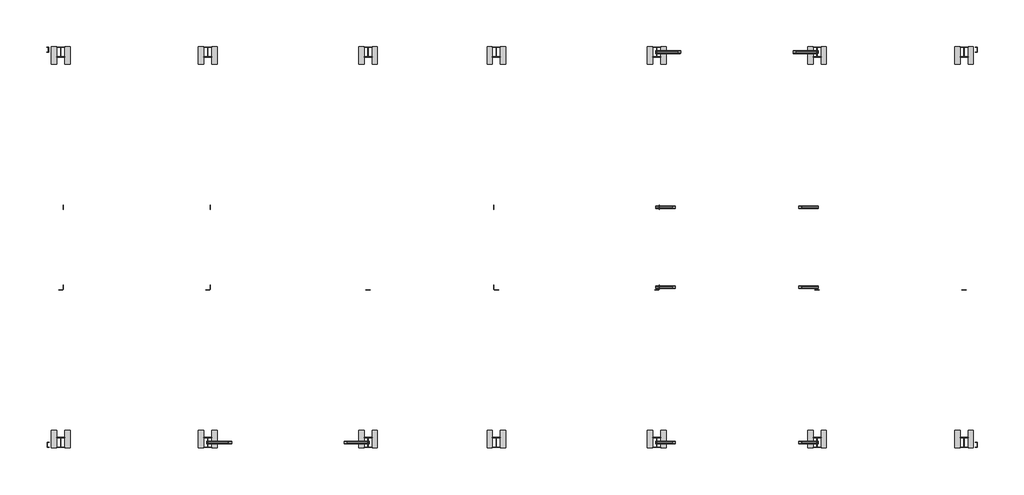
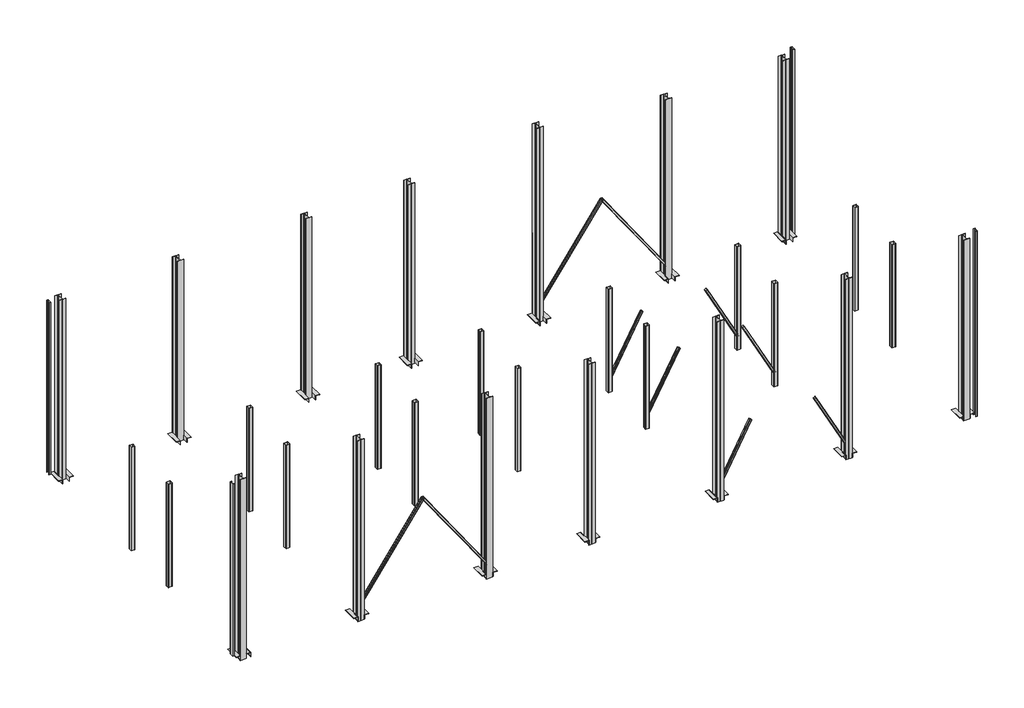
# One storey: 56 beams, 14 columns.
"""IFC4 building model written with IfcOpenShell, lengths in millimetres."""

import ifcopenshell
import ifcopenshell.guid

model = None  # the IFC model being written
_history = None  # IfcOwnerHistory: only IFC2X3 demands one
_inside = {}  # id of a spatial element -> (the spatial element, [elements in it])
_under = {}  # id of a project, library or spatial element -> (it, [spatial elements below it])
_declared = {}  # id of a project -> (the project, [libraries it declares])
_typed = {}  # id of a type object -> (the type object, [elements of that type])
_made_of = {}  # id of a material, layer set ... -> (it, [elements and type objects made of it])


def new_model(schema):
    """Start an empty IFC model of exactly this schema.

    Asked for "IFC4X3", IfcOpenShell would pick the latest addendum, in which some entities
    have other attributes; the version numbers below select the first issue.
    IFC2X3 requires an IfcOwnerHistory on every rooted entity: one is made here for all.
    """
    global model, _history
    if schema == "IFC4X3":
        model = ifcopenshell.file(schema_version=(4, 3, 0, 0))
    else:
        model = ifcopenshell.file(schema=schema)
    _inside.clear()
    _under.clear()
    _declared.clear()
    _typed.clear()
    _made_of.clear()
    _history = None
    if model.schema == "IFC2X3":
        org = make("IfcOrganization", Name="unknown")
        user = make(
            "IfcPersonAndOrganization",
            ThePerson=make("IfcPerson", FamilyName="unknown"),
            TheOrganization=org,
        )
        app = make(
            "IfcApplication",
            ApplicationDeveloper=org,
            Version="unknown",
            ApplicationFullName="unknown",
            ApplicationIdentifier="unknown",
        )
        _history = make(
            "IfcOwnerHistory",
            OwningUser=user,
            OwningApplication=app,
            ChangeAction="ADDED",
            CreationDate=0,
        )
    return model


def make(cls, **values):
    """One entity of the class cls with the attributes given. An attribute that is None is left unset."""
    return model.create_entity(
        cls, **{name: value for name, value in values.items() if value is not None}
    )


def rooted(cls, **values):
    """An entity with a GlobalId (a new one), such as an element, a storey or a relation."""
    return make(cls, GlobalId=ifcopenshell.guid.new(), OwnerHistory=_history, **values)


def si_unit(unit_type, name, prefix=None):
    """IfcSIUnit, for example si_unit("LENGTHUNIT", "METRE", prefix="MILLI")."""
    return make("IfcSIUnit", UnitType=unit_type, Prefix=prefix, Name=name)


def assignment(units):
    """IfcUnitAssignment: the units of a project."""
    return None if units is None else make("IfcUnitAssignment", Units=units)


def point(xyz):
    """IfcCartesianPoint."""
    return None if xyz is None else make("IfcCartesianPoint", Coordinates=xyz)


def direction(xyz):
    """IfcDirection."""
    return None if xyz is None else make("IfcDirection", DirectionRatios=xyz)


def frame(location, z_axis=None, x_axis=None):
    """IfcAxis2Placement3D, a coordinate frame: its origin and axes. An axis left out is left unset."""
    return make(
        "IfcAxis2Placement3D",
        Location=point(location),
        Axis=direction(z_axis),
        RefDirection=direction(x_axis),
    )


def frame_2d(location, x_axis=None):
    """IfcAxis2Placement2D, a coordinate frame in the plane: its origin and x axis."""
    return make(
        "IfcAxis2Placement2D", Location=point(location), RefDirection=direction(x_axis)
    )


def origin():
    """The frame at (0, 0, 0) with its axes left unset."""
    return frame((0.0, 0.0, 0.0))


def origin_with_axes():
    """The frame at (0, 0, 0) with the z axis (0, 0, 1) and the x axis (1, 0, 0) written out."""
    return frame((0.0, 0.0, 0.0), z_axis=(0.0, 0.0, 1.0), x_axis=(1.0, 0.0, 0.0))


def place(relative_to, where):
    """IfcLocalPlacement: puts the frame where relative to a parent placement (None: the world)."""
    return make(
        "IfcLocalPlacement", PlacementRelTo=relative_to, RelativePlacement=where
    )


def context(
    kind, dimensions, precision=None, world=None, true_north=None, identifier=None
):
    """IfcGeometricRepresentationContext, for example the 3D "Model" context."""
    return make(
        "IfcGeometricRepresentationContext",
        ContextIdentifier=identifier,
        ContextType=kind,
        CoordinateSpaceDimension=dimensions,
        Precision=precision,
        WorldCoordinateSystem=world,
        TrueNorth=true_north,
    )


def project(units=None, contexts=None):
    """IfcProject with its units and contexts."""
    return rooted(
        "IfcProject",
        Name="project",
        RepresentationContexts=contexts,
        UnitsInContext=assignment(units),
    )


def spatial(cls, under=None, at=None, **own):
    """A site, building, storey or space (cls), placed at a placement, below another one or the project."""
    s = rooted(cls, ObjectPlacement=at, **own)
    if under is not None:
        _under.setdefault(under.id(), (under, []))[1].append(s)
    return s


def polyline(points):
    """IfcPolyline through the points."""
    return make("IfcPolyline", Points=[point(p) for p in points])


def circle_curve(where, radius):
    """IfcCircle in the frame where."""
    return make("IfcCircle", Position=where, Radius=radius)


def trimmed(basis, trim1, trim2, sense, master):
    """IfcTrimmedCurve: the piece of a basis curve between two trims."""
    return make(
        "IfcTrimmedCurve",
        BasisCurve=basis,
        Trim1=trim1,
        Trim2=trim2,
        SenseAgreement=sense,
        MasterRepresentation=master,
    )


def segment(curve, same_sense, transition):
    """IfcCompositeCurveSegment."""
    return make(
        "IfcCompositeCurveSegment",
        Transition=transition,
        SameSense=same_sense,
        ParentCurve=curve,
    )


def composite_curve(segments, self_intersect=None):
    """IfcCompositeCurve: segments joined end to end."""
    return make("IfcCompositeCurve", Segments=segments, SelfIntersect=self_intersect)


def outline(outer, holes=None, kind="AREA"):
    """IfcArbitraryClosedProfileDef: a profile drawn as a closed curve; with holes, ...WithVoids."""
    if holes is None:
        return make("IfcArbitraryClosedProfileDef", ProfileType=kind, OuterCurve=outer)
    return make(
        "IfcArbitraryProfileDefWithVoids",
        ProfileType=kind,
        OuterCurve=outer,
        InnerCurves=holes,
    )


def extrude(swept, where, along, depth):
    """IfcExtrudedAreaSolid: the profile swept, set in the frame where, extruded along a direction by depth."""
    return make(
        "IfcExtrudedAreaSolid",
        SweptArea=swept,
        Position=where,
        ExtrudedDirection=direction(along),
        Depth=depth,
    )


def shape(context_of_items, identifier, shape_type, items):
    """IfcShapeRepresentation: the items that make up one representation, for example the "Body"."""
    return make(
        "IfcShapeRepresentation",
        ContextOfItems=context_of_items,
        RepresentationIdentifier=identifier,
        RepresentationType=shape_type,
        Items=items,
    )


def source(mapping_origin, context_of_items, identifier, shape_type, items):
    """IfcRepresentationMap: a shape defined once, which mapped items show again and again."""
    return make(
        "IfcRepresentationMap",
        MappingOrigin=mapping_origin,
        MappedRepresentation=shape(context_of_items, identifier, shape_type, items),
    )


def transform(
    local_origin,
    x_axis=None,
    y_axis=None,
    z_axis=None,
    scale=None,
    scale2=None,
    scale3=None,
    uniform=True,
):
    """IfcCartesianTransformationOperator3D, or its non-uniform kind. x_axis, y_axis, z_axis: its Axis1, 2, 3."""
    if uniform:
        return make(
            "IfcCartesianTransformationOperator3D",
            Axis1=direction(x_axis),
            Axis2=direction(y_axis),
            LocalOrigin=point(local_origin),
            Scale=scale,
            Axis3=direction(z_axis),
        )
    return make(
        "IfcCartesianTransformationOperator3DnonUniform",
        Axis1=direction(x_axis),
        Axis2=direction(y_axis),
        LocalOrigin=point(local_origin),
        Scale=scale,
        Axis3=direction(z_axis),
        Scale2=scale2,
        Scale3=scale3,
    )


def mapped(mapping_source, mapping_target):
    """IfcMappedItem: shows the shape of a source again, moved by a transform."""
    return make(
        "IfcMappedItem", MappingSource=mapping_source, MappingTarget=mapping_target
    )


def made_of(thing, what):
    """Note that an element or type object is made of a material, layer set ...; save() writes the relation."""
    if what is not None:
        _made_of.setdefault(what.id(), (what, []))[1].append(thing)
    return thing


def element(
    cls,
    number,
    at=None,
    inside=None,
    cuts=None,
    type_object=None,
    material=None,
    context=None,
    identifier="Body",
    shape_type=None,
    held_by="IfcProductDefinitionShape",
    body=None,
    shapes=None,
    **own,
):
    """One element of the class cls, such as IfcWall. Its Tag is "e" and its number.

    at: its placement. inside: the storey or other place that contains it. cuts: it is an
    opening in that element (IfcRelVoidsElement). A single representation is given by context,
    identifier, shape_type and body (its items); several are given by shapes. held_by: the class
    of the entity that holds the representations. save() writes the other relations.
    """
    e = rooted(cls, Tag="e%d" % number, ObjectPlacement=at, **own)
    if body is not None:
        shapes = [shape(context, identifier, shape_type, body)]
    if shapes is not None:
        e.Representation = make(held_by, Representations=shapes)
    if inside is not None:
        _inside.setdefault(inside.id(), (inside, []))[1].append(e)
    if cuts is not None:
        rooted(
            "IfcRelVoidsElement", RelatingBuildingElement=cuts, RelatedOpeningElement=e
        )
    if type_object is not None:
        _typed.setdefault(type_object.id(), (type_object, []))[1].append(e)
    return made_of(e, material)


def aggregate(whole, parts):
    """IfcRelAggregates: a whole, such as a stair, and the parts it consists of."""
    return rooted("IfcRelAggregates", RelatingObject=whole, RelatedObjects=parts)


def save(model, path):
    """Write the relations noted so far, then the file.

    IfcRelAggregates (storeys below a building ...), IfcRelContainedInSpatialStructure (elements
    in a storey), IfcRelDefinesByType, IfcRelAssociatesMaterial and IfcRelDeclares: one each for
    every whole, place, type object, material and project.
    """
    for whole, parts in _under.values():
        aggregate(whole, parts)
    for where, things in _inside.values():
        rooted(
            "IfcRelContainedInSpatialStructure",
            RelatedElements=things,
            RelatingStructure=where,
        )
    for kind, things in _typed.values():
        rooted("IfcRelDefinesByType", RelatedObjects=things, RelatingType=kind)
    for what, things in _made_of.values():
        rooted("IfcRelAssociatesMaterial", RelatedObjects=things, RelatingMaterial=what)
    for by, libraries in _declared.values():
        rooted("IfcRelDeclares", RelatingContext=by, RelatedDefinitions=libraries)
    model.write(path)


def beam_75da4e79(model_context):
    return source(origin(), model_context, "Body", "SweptSolid", [
        extrude(outline(composite_curve([segment(polyline([(-78.0, 90.0), (78.0, 90.0)]), True, "CONTINUOUS"), segment(trimmed(circle_curve(frame_2d((78.0, 78.0)), 12.0), [point((78.0, 90.0))], [point((90.0, 78.0))], False, "CARTESIAN"), True, "CONTINUOUS"), segment(polyline([(90.0, 78.0), (90.0, -78.0)]), True, "CONTINUOUS"), segment(trimmed(circle_curve(frame_2d((78.0, -78.0)), 12.0), [point((90.0, -78.0))], [point((78.0, -90.0))], False, "CARTESIAN"), True, "CONTINUOUS"), segment(polyline([(78.0, -90.0), (-78.0, -90.0)]), True, "CONTINUOUS"), segment(trimmed(circle_curve(frame_2d((-78.0, -78.0)), 12.0), [point((-78.0, -90.0))], [point((-90.0, -78.0))], False, "CARTESIAN"), True, "CONTINUOUS"), segment(polyline([(-90.0, -78.0), (-90.0, 78.0)]), True, "CONTINUOUS"), segment(trimmed(circle_curve(frame_2d((-78.0, 78.0)), 12.0), [point((-90.0, 78.0))], [point((-78.0, 90.0))], False, "CARTESIAN"), True, "CONTINUOUS")], self_intersect=False), holes=[composite_curve([segment(trimmed(circle_curve(frame_2d((-78.0, 78.0)), 6.0), [point((-78.0, 84.0))], [point((-84.0, 78.0))], True, "CARTESIAN"), True, "CONTINUOUS"), segment(polyline([(-84.0, 78.0), (-84.0, -78.0)]), True, "CONTINUOUS"), segment(trimmed(circle_curve(frame_2d((-78.0, -78.0)), 6.0), [point((-84.0, -78.0))], [point((-78.0, -84.0))], True, "CARTESIAN"), True, "CONTINUOUS"), segment(polyline([(-78.0, -84.0), (78.0, -84.0)]), True, "CONTINUOUS"), segment(trimmed(circle_curve(frame_2d((78.0, -78.0)), 6.0), [point((78.0, -84.0))], [point((84.0, -78.0))], True, "CARTESIAN"), True, "CONTINUOUS"), segment(polyline([(84.0, -78.0), (84.0, 78.0)]), True, "CONTINUOUS"), segment(trimmed(circle_curve(frame_2d((78.0, 78.0)), 6.0), [point((84.0, 78.0))], [point((78.0, 84.0))], True, "CARTESIAN"), True, "CONTINUOUS"), segment(polyline([(78.0, 84.0), (-78.0, 84.0)]), True, "CONTINUOUS")], self_intersect=False)]), frame((-2550.0, 0.0, 0.0), z_axis=(1.0, 0.0, 0.0), x_axis=(0.0, 1.0, 0.0)), (0.0, 0.0, 1.0), 5100.0),
    ])


def beam_97961db2(model_context):
    return source(origin(), model_context, "Body", "SweptSolid", [
        extrude(outline(composite_curve([segment(polyline([(23.0, 100.0), (23.0, -100.0), (-53.0, -100.0), (-53.0, -91.0), (8.3, -91.0)]), True, "CONTINUOUS"), segment(trimmed(circle_curve(frame_2d((8.3, -81.5)), 9.5), [point((8.3, -91.0))], [point((17.8, -81.5))], True, "CARTESIAN"), True, "CONTINUOUS"), segment(polyline([(17.8, -81.5), (17.8, 81.5)]), True, "CONTINUOUS"), segment(trimmed(circle_curve(frame_2d((8.3, 81.5)), 9.5), [point((17.8, 81.5))], [point((8.3, 91.0))], True, "CARTESIAN"), True, "CONTINUOUS"), segment(polyline([(8.3, 91.0), (-53.0, 91.0), (-53.0, 100.0), (23.0, 100.0)]), True, "CONTINUOUS")], self_intersect=False)), frame((-4250.0, 0.0, 0.0), z_axis=(1.0, 0.0, 0.0), x_axis=(0.0, 1.0, 0.0)), (0.0, 0.0, 1.0), 8500.0),
    ])


def beam_6aa5ee4f(model_context):
    return source(origin(), model_context, "Body", "SweptSolid", [
        extrude(outline(composite_curve([segment(polyline([(-38.0, 50.0), (38.0, 50.0)]), True, "CONTINUOUS"), segment(trimmed(circle_curve(frame_2d((38.0, 38.0)), 12.0), [point((38.0, 50.0))], [point((50.0, 38.0))], False, "CARTESIAN"), True, "CONTINUOUS"), segment(polyline([(50.0, 38.0), (50.0, -38.0)]), True, "CONTINUOUS"), segment(trimmed(circle_curve(frame_2d((38.0, -38.0)), 12.0), [point((50.0, -38.0))], [point((38.0, -50.0))], False, "CARTESIAN"), True, "CONTINUOUS"), segment(polyline([(38.0, -50.0), (-38.0, -50.0)]), True, "CONTINUOUS"), segment(trimmed(circle_curve(frame_2d((-38.0, -38.0)), 12.0), [point((-38.0, -50.0))], [point((-50.0, -38.0))], False, "CARTESIAN"), True, "CONTINUOUS"), segment(polyline([(-50.0, -38.0), (-50.0, 38.0)]), True, "CONTINUOUS"), segment(trimmed(circle_curve(frame_2d((-38.0, 38.0)), 12.0), [point((-50.0, 38.0))], [point((-38.0, 50.0))], False, "CARTESIAN"), True, "CONTINUOUS")], self_intersect=False), holes=[composite_curve([segment(trimmed(circle_curve(frame_2d((-38.0, 38.0)), 6.0), [point((-38.0, 44.0))], [point((-44.0, 38.0))], True, "CARTESIAN"), True, "CONTINUOUS"), segment(polyline([(-44.0, 38.0), (-44.0, -38.0)]), True, "CONTINUOUS"), segment(trimmed(circle_curve(frame_2d((-38.0, -38.0)), 6.0), [point((-44.0, -38.0))], [point((-38.0, -44.0))], True, "CARTESIAN"), True, "CONTINUOUS"), segment(polyline([(-38.0, -44.0), (38.0, -44.0)]), True, "CONTINUOUS"), segment(trimmed(circle_curve(frame_2d((38.0, -38.0)), 6.0), [point((38.0, -44.0))], [point((44.0, -38.0))], True, "CARTESIAN"), True, "CONTINUOUS"), segment(polyline([(44.0, -38.0), (44.0, 38.0)]), True, "CONTINUOUS"), segment(trimmed(circle_curve(frame_2d((38.0, 38.0)), 6.0), [point((44.0, 38.0))], [point((38.0, 44.0))], True, "CARTESIAN"), True, "CONTINUOUS"), segment(polyline([(38.0, 44.0), (-38.0, 44.0)]), True, "CONTINUOUS")], self_intersect=False)]), frame((-2618.5, 0.0, 0.0), z_axis=(1.0, 0.0, 0.0), x_axis=(0.0, 1.0, 0.0)), (0.0, 0.0, 1.0), 5237.0),
    ])


def beam_810e5c83(model_context):
    return source(origin(), model_context, "Body", "SweptSolid", [
        extrude(outline(composite_curve([segment(polyline([(-38.0, 50.0), (38.0, 50.0)]), True, "CONTINUOUS"), segment(trimmed(circle_curve(frame_2d((38.0, 38.0)), 12.0), [point((38.0, 50.0))], [point((50.0, 38.0))], False, "CARTESIAN"), True, "CONTINUOUS"), segment(polyline([(50.0, 38.0), (50.0, -38.0)]), True, "CONTINUOUS"), segment(trimmed(circle_curve(frame_2d((38.0, -38.0)), 12.0), [point((50.0, -38.0))], [point((38.0, -50.0))], False, "CARTESIAN"), True, "CONTINUOUS"), segment(polyline([(38.0, -50.0), (-38.0, -50.0)]), True, "CONTINUOUS"), segment(trimmed(circle_curve(frame_2d((-38.0, -38.0)), 12.0), [point((-38.0, -50.0))], [point((-50.0, -38.0))], False, "CARTESIAN"), True, "CONTINUOUS"), segment(polyline([(-50.0, -38.0), (-50.0, 38.0)]), True, "CONTINUOUS"), segment(trimmed(circle_curve(frame_2d((-38.0, 38.0)), 12.0), [point((-50.0, 38.0))], [point((-38.0, 50.0))], False, "CARTESIAN"), True, "CONTINUOUS")], self_intersect=False), holes=[composite_curve([segment(trimmed(circle_curve(frame_2d((-38.0, 38.0)), 6.0), [point((-38.0, 44.0))], [point((-44.0, 38.0))], True, "CARTESIAN"), True, "CONTINUOUS"), segment(polyline([(-44.0, 38.0), (-44.0, -38.0)]), True, "CONTINUOUS"), segment(trimmed(circle_curve(frame_2d((-38.0, -38.0)), 6.0), [point((-44.0, -38.0))], [point((-38.0, -44.0))], True, "CARTESIAN"), True, "CONTINUOUS"), segment(polyline([(-38.0, -44.0), (38.0, -44.0)]), True, "CONTINUOUS"), segment(trimmed(circle_curve(frame_2d((38.0, -38.0)), 6.0), [point((38.0, -44.0))], [point((44.0, -38.0))], True, "CARTESIAN"), True, "CONTINUOUS"), segment(polyline([(44.0, -38.0), (44.0, 38.0)]), True, "CONTINUOUS"), segment(trimmed(circle_curve(frame_2d((38.0, 38.0)), 6.0), [point((44.0, 38.0))], [point((38.0, 44.0))], True, "CARTESIAN"), True, "CONTINUOUS"), segment(polyline([(38.0, 44.0), (-38.0, 44.0)]), True, "CONTINUOUS")], self_intersect=False)]), frame((-1601.0, 0.0, 0.0), z_axis=(1.0, 0.0, 0.0), x_axis=(0.0, 1.0, 0.0)), (0.0, 0.0, 1.0), 3202.0),
    ])


def beam_48740a10(model_context):
    return source(origin(), model_context, "Body", "SweptSolid", [
        extrude(outline(composite_curve([segment(polyline([(-23.0, 100.0), (53.0, 100.0), (53.0, 91.0), (-8.3, 91.0)]), True, "CONTINUOUS"), segment(trimmed(circle_curve(frame_2d((-8.3, 81.5)), 9.5), [point((-8.3, 91.0))], [point((-17.8, 81.5))], True, "CARTESIAN"), True, "CONTINUOUS"), segment(polyline([(-17.8, 81.5), (-17.8, -81.5)]), True, "CONTINUOUS"), segment(trimmed(circle_curve(frame_2d((-8.3, -81.5)), 9.5), [point((-17.8, -81.5))], [point((-8.3, -91.0))], True, "CARTESIAN"), True, "CONTINUOUS"), segment(polyline([(-8.3, -91.0), (53.0, -91.0), (53.0, -100.0), (-23.0, -100.0), (-23.0, 100.0)]), True, "CONTINUOUS")], self_intersect=False)), frame((-4585.0, 0.0, 0.0), z_axis=(1.0, 0.0, 0.0), x_axis=(0.0, 1.0, 0.0)), (0.0, 0.0, 1.0), 9170.0),
    ])


def beam_e8fb0e59(model_context):
    return source(origin(), model_context, "Body", "SweptSolid", [
        extrude(outline(composite_curve([segment(polyline([(23.0, 100.0), (23.0, -100.0), (-53.0, -100.0), (-53.0, -91.0), (8.3, -91.0)]), True, "CONTINUOUS"), segment(trimmed(circle_curve(frame_2d((8.3, -81.5)), 9.5), [point((8.3, -91.0))], [point((17.8, -81.5))], True, "CARTESIAN"), True, "CONTINUOUS"), segment(polyline([(17.8, -81.5), (17.8, 81.5)]), True, "CONTINUOUS"), segment(trimmed(circle_curve(frame_2d((8.3, 81.5)), 9.5), [point((17.8, 81.5))], [point((8.3, 91.0))], True, "CARTESIAN"), True, "CONTINUOUS"), segment(polyline([(8.3, 91.0), (-53.0, 91.0), (-53.0, 100.0), (23.0, 100.0)]), True, "CONTINUOUS")], self_intersect=False)), frame((-4585.0, 0.0, 0.0), z_axis=(1.0, 0.0, 0.0), x_axis=(0.0, 1.0, 0.0)), (0.0, 0.0, 1.0), 9170.0),
    ])


def l_200x14_1023fe27(model_context):
    return source(origin(), model_context, "Body", "SweptSolid", [
        extrude(outline(composite_curve([segment(polyline([(54.6, -54.6), (-145.4, -54.6), (-145.4, -46.6)]), True, "CONTINUOUS"), segment(trimmed(circle_curve(frame_2d((-139.4, -46.6)), 6.0), [point((-145.4, -46.6))], [point((-139.4, -40.6))], False, "CARTESIAN"), True, "CONTINUOUS"), segment(polyline([(-139.4, -40.6), (22.6, -40.6)]), True, "CONTINUOUS"), segment(trimmed(circle_curve(frame_2d((22.6, -22.6)), 18.0), [point((22.6, -40.6))], [point((40.6, -22.6))], True, "CARTESIAN"), True, "CONTINUOUS"), segment(polyline([(40.6, -22.6), (40.6, 139.4)]), True, "CONTINUOUS"), segment(trimmed(circle_curve(frame_2d((46.6, 139.4)), 6.0), [point((40.6, 139.4))], [point((46.6, 145.4))], False, "CARTESIAN"), True, "CONTINUOUS"), segment(polyline([(46.6, 145.4), (54.6, 145.4), (54.6, -54.6)]), True, "CONTINUOUS")], self_intersect=False)), frame((-335.0, 0.0, 0.0), z_axis=(1.0, 0.0, 0.0), x_axis=(0.0, 1.0, 0.0)), (0.0, 0.0, 1.0), 670.0),
    ])


def l_200x14_4beb5e8d(model_context):
    return source(origin(), model_context, "Body", "SweptSolid", [
        extrude(outline(composite_curve([segment(polyline([(-54.6, -54.6), (-54.6, 145.4), (-46.6, 145.4)]), True, "CONTINUOUS"), segment(trimmed(circle_curve(frame_2d((-46.6, 139.4)), 6.0), [point((-46.6, 145.4))], [point((-40.6, 139.4))], False, "CARTESIAN"), True, "CONTINUOUS"), segment(polyline([(-40.6, 139.4), (-40.6, -22.6)]), True, "CONTINUOUS"), segment(trimmed(circle_curve(frame_2d((-22.6, -22.6)), 18.0), [point((-40.6, -22.6))], [point((-22.6, -40.6))], True, "CARTESIAN"), True, "CONTINUOUS"), segment(polyline([(-22.6, -40.6), (139.4, -40.6)]), True, "CONTINUOUS"), segment(trimmed(circle_curve(frame_2d((139.4, -46.6)), 6.0), [point((139.4, -40.6))], [point((145.4, -46.6))], False, "CARTESIAN"), True, "CONTINUOUS"), segment(polyline([(145.4, -46.6), (145.4, -54.6), (-54.6, -54.6)]), True, "CONTINUOUS")], self_intersect=False)), frame((-335.0, 0.0, 0.0), z_axis=(1.0, 0.0, 0.0), x_axis=(0.0, 1.0, 0.0)), (0.0, 0.0, 1.0), 670.0),
    ])


def i_40h1_838be756(model_context):
    return source(origin(), model_context, "Body", "SweptSolid", [
        extrude(outline(composite_curve([segment(polyline([(-149.5, -178.5), (-26.75, -178.5)]), True, "CONTINUOUS"), segment(trimmed(circle_curve(frame_2d((-26.75, -156.5)), 22.0), [point((-26.75, -178.5))], [point((-4.75, -156.5))], True, "CARTESIAN"), True, "CONTINUOUS"), segment(polyline([(-4.75, -156.5), (-4.75, 157.5)]), True, "CONTINUOUS"), segment(trimmed(circle_curve(frame_2d((-26.75, 157.5)), 22.0), [point((-4.75, 157.5))], [point((-26.75, 179.5))], True, "CARTESIAN"), True, "CONTINUOUS"), segment(polyline([(-26.75, 179.5), (-149.5, 179.5), (-149.5, 192.0), (149.5, 192.0), (149.5, 179.5), (26.75, 179.5)]), True, "CONTINUOUS"), segment(trimmed(circle_curve(frame_2d((26.75, 157.5)), 22.0), [point((26.75, 179.5))], [point((4.75, 157.5))], True, "CARTESIAN"), True, "CONTINUOUS"), segment(polyline([(4.75, 157.5), (4.75, -156.5)]), True, "CONTINUOUS"), segment(trimmed(circle_curve(frame_2d((26.75, -156.5)), 22.0), [point((4.75, -156.5))], [point((26.75, -178.5))], True, "CARTESIAN"), True, "CONTINUOUS"), segment(polyline([(26.75, -178.5), (149.5, -178.5), (149.5, -191.0), (-149.5, -191.0), (-149.5, -178.5)]), True, "CONTINUOUS")], self_intersect=False)), origin_with_axes(), (0.0, 0.0, 1.0), 9604.6332616),
    ])


def i_40h1_0f399548(model_context):
    return source(origin(), model_context, "Body", "SweptSolid", [
        extrude(outline(composite_curve([segment(polyline([(-149.5, 178.5), (-149.5, 191.0), (149.5, 191.0), (149.5, 178.5), (26.75, 178.5)]), True, "CONTINUOUS"), segment(trimmed(circle_curve(frame_2d((26.75, 156.5)), 22.0), [point((26.75, 178.5))], [point((4.75, 156.5))], True, "CARTESIAN"), True, "CONTINUOUS"), segment(polyline([(4.75, 156.5), (4.75, -157.5)]), True, "CONTINUOUS"), segment(trimmed(circle_curve(frame_2d((26.75, -157.5)), 22.0), [point((4.75, -157.5))], [point((26.75, -179.5))], True, "CARTESIAN"), True, "CONTINUOUS"), segment(polyline([(26.75, -179.5), (149.5, -179.5), (149.5, -192.0), (-149.5, -192.0), (-149.5, -179.5), (-26.75, -179.5)]), True, "CONTINUOUS"), segment(trimmed(circle_curve(frame_2d((-26.75, -157.5)), 22.0), [point((-26.75, -179.5))], [point((-4.75, -157.5))], True, "CARTESIAN"), True, "CONTINUOUS"), segment(polyline([(-4.75, -157.5), (-4.75, 156.5)]), True, "CONTINUOUS"), segment(trimmed(circle_curve(frame_2d((-26.75, 156.5)), 22.0), [point((-4.75, 156.5))], [point((-26.75, 178.5))], True, "CARTESIAN"), True, "CONTINUOUS"), segment(polyline([(-26.75, 178.5), (-149.5, 178.5)]), True, "CONTINUOUS")], self_intersect=False)), origin_with_axes(), (0.0, 0.0, 1.0), 8923.3858447),
    ])


def i_40h1_edde52e3(model_context):
    return source(origin(), model_context, "Body", "SweptSolid", [
        extrude(outline(composite_curve([segment(polyline([(-149.5, -178.5), (-26.75, -178.5)]), True, "CONTINUOUS"), segment(trimmed(circle_curve(frame_2d((-26.75, -156.5)), 22.0), [point((-26.75, -178.5))], [point((-4.75, -156.5))], True, "CARTESIAN"), True, "CONTINUOUS"), segment(polyline([(-4.75, -156.5), (-4.75, 157.5)]), True, "CONTINUOUS"), segment(trimmed(circle_curve(frame_2d((-26.75, 157.5)), 22.0), [point((-4.75, 157.5))], [point((-26.75, 179.5))], True, "CARTESIAN"), True, "CONTINUOUS"), segment(polyline([(-26.75, 179.5), (-149.5, 179.5), (-149.5, 192.0), (149.5, 192.0), (149.5, 179.5), (26.75, 179.5)]), True, "CONTINUOUS"), segment(trimmed(circle_curve(frame_2d((26.75, 157.5)), 22.0), [point((26.75, 179.5))], [point((4.75, 157.5))], True, "CARTESIAN"), True, "CONTINUOUS"), segment(polyline([(4.75, 157.5), (4.75, -156.5)]), True, "CONTINUOUS"), segment(trimmed(circle_curve(frame_2d((26.75, -156.5)), 22.0), [point((4.75, -156.5))], [point((26.75, -178.5))], True, "CARTESIAN"), True, "CONTINUOUS"), segment(polyline([(26.75, -178.5), (149.5, -178.5), (149.5, -191.0), (-149.5, -191.0), (-149.5, -178.5)]), True, "CONTINUOUS")], self_intersect=False)), origin_with_axes(), (0.0, 0.0, 1.0), 8923.3858447),
    ])


model = new_model("IFC4")

# Units and contexts
model_context = context("Model", 3, world=origin())
ifc_project = project(units=[si_unit("LENGTHUNIT", "METRE", prefix="MILLI")], contexts=[model_context])

# Site, building, storey
site = spatial("IfcSite", under=ifc_project)
building = spatial("IfcBuilding", under=site)
storey = spatial("IfcBuildingStorey", under=building, Name="Этаж 01", Elevation=0.0)

# Beams
placement = place(None, origin())
beam_shape = beam_75da4e79(model_context)
element("IfcBeam", 1, ObjectType="Гнутый прямоугольный профиль (Трубы 30245-94) Балки : гнутый прямоуг. проф. 180x6", at=placement, inside=storey, context=model_context, shape_type="MappedRepresentation", body=[
    mapped(beam_shape, transform((6000.0, 9000.0, 1950.0), x_axis=(0.0, 0.0, 1.0), y_axis=(0.0, -1.0, 0.0), z_axis=(1.0, 0.0, 0.0))),
])
element("IfcBeam", 2, ObjectType="Гнутый прямоугольный профиль (Трубы 30245-94) Балки : гнутый прямоуг. проф. 180x6", at=placement, inside=storey, context=model_context, shape_type="MappedRepresentation", body=[
    mapped(beam_shape, transform((6000.0, 6000.0, 1950.0), x_axis=(0.0, 0.0, 1.0), y_axis=(0.0, -1.0, 0.0), z_axis=(1.0, 0.0, 0.0))),
])
element("IfcBeam", 3, ObjectType="Гнутый прямоугольный профиль (Трубы 30245-94) Балки : гнутый прямоуг. проф. 180x6", at=placement, inside=storey, context=model_context, shape_type="MappedRepresentation", body=[
    mapped(beam_shape, transform((12000.0, 9000.0, 1950.0), x_axis=(0.0, 0.0, 1.0), y_axis=(0.0, -1.0, 0.0), z_axis=(1.0, 0.0, 0.0))),
])
element("IfcBeam", 4, ObjectType="Гнутый прямоугольный профиль (Трубы 30245-94) Балки : гнутый прямоуг. проф. 180x6", at=placement, inside=storey, context=model_context, shape_type="MappedRepresentation", body=[
    mapped(beam_shape, transform((12000.0, 6000.0, 1950.0), x_axis=(0.0, 0.0, 1.0), y_axis=(0.0, -1.0, 0.0), z_axis=(1.0, 0.0, 0.0))),
])
element("IfcBeam", 5, ObjectType="Гнутый прямоугольный профиль (Трубы 30245-94) Балки : гнутый прямоуг. проф. 180x6", at=placement, inside=storey, context=model_context, shape_type="MappedRepresentation", body=[
    mapped(beam_shape, transform((16800.0, 9000.0, 1950.0), x_axis=(0.0, 0.0, 1.0), y_axis=(0.0, -1.0, 0.0), z_axis=(1.0, 0.0, 0.0))),
])
element("IfcBeam", 6, ObjectType="Гнутый прямоугольный профиль (Трубы 30245-94) Балки : гнутый прямоуг. проф. 180x6", at=placement, inside=storey, context=model_context, shape_type="MappedRepresentation", body=[
    mapped(beam_shape, transform((16800.0, 6000.0, 1950.0), x_axis=(0.0, 0.0, 1.0), y_axis=(0.0, -1.0, 0.0), z_axis=(1.0, 0.0, 0.0))),
])
element("IfcBeam", 7, ObjectType="Гнутый прямоугольный профиль (Трубы 30245-94) Балки : гнутый прямоуг. проф. 180x6", at=placement, inside=storey, context=model_context, shape_type="MappedRepresentation", body=[
    mapped(beam_shape, transform((22800.0, 9000.0, 1950.0), x_axis=(0.0, 0.0, 1.0), y_axis=(0.0, -1.0, 0.0), z_axis=(1.0, 0.0, 0.0))),
])
element("IfcBeam", 8, ObjectType="Гнутый прямоугольный профиль (Трубы 30245-94) Балки : гнутый прямоуг. проф. 180x6", at=placement, inside=storey, context=model_context, shape_type="MappedRepresentation", body=[
    mapped(beam_shape, transform((22800.0, 6000.0, 1950.0), x_axis=(0.0, 0.0, 1.0), y_axis=(0.0, -1.0, 0.0), z_axis=(1.0, 0.0, 0.0))),
])
element("IfcBeam", 9, ObjectType="Гнутый прямоугольный профиль (Трубы 30245-94) Балки : гнутый прямоуг. проф. 180x6", at=placement, inside=storey, context=model_context, shape_type="MappedRepresentation", body=[
    mapped(beam_shape, transform((28800.0, 6000.0, 1950.0), x_axis=(0.0, 0.0, 1.0), y_axis=(0.0, -1.0, 0.0), z_axis=(1.0, 0.0, 0.0))),
])
element("IfcBeam", 10, ObjectType="Гнутый прямоугольный профиль (Трубы 30245-94) Балки : гнутый прямоуг. проф. 180x6", at=placement, inside=storey, context=model_context, shape_type="MappedRepresentation", body=[
    mapped(beam_shape, transform((28800.0, 9000.0, 1950.0), x_axis=(0.0, 0.0, 1.0), y_axis=(0.0, -1.0, 0.0), z_axis=(1.0, 0.0, 0.0))),
])
element("IfcBeam", 11, ObjectType="Гнутый прямоугольный профиль (Трубы 30245-94) Балки : гнутый прямоуг. проф. 180x6", at=placement, inside=storey, context=model_context, shape_type="MappedRepresentation", body=[
    mapped(beam_shape, transform((34300.0, 9000.0, 1950.0), x_axis=(0.0, 0.0, 1.0), y_axis=(0.0, -1.0, 0.0), z_axis=(1.0, 0.0, 0.0))),
])
element("IfcBeam", 12, ObjectType="Гнутый прямоугольный профиль (Трубы 30245-94) Балки : гнутый прямоуг. проф. 180x6", at=placement, inside=storey, context=model_context, shape_type="MappedRepresentation", body=[
    mapped(beam_shape, transform((34300.0, 6000.0, 1950.0), x_axis=(0.0, 0.0, 1.0), y_axis=(0.0, -1.0, 0.0), z_axis=(1.0, 0.0, 0.0))),
])
element("IfcBeam", 13, ObjectType="Гнутый прямоугольный профиль (Трубы 30245-94) Балки : гнутый прямоуг. проф. 180x6", at=placement, inside=storey, context=model_context, shape_type="MappedRepresentation", body=[
    mapped(beam_shape, transform((500.0, 9000.0, 1950.0), x_axis=(0.0, 0.0, 1.0), y_axis=(0.0, -1.0, 0.0), z_axis=(1.0, 0.0, 0.0))),
])
element("IfcBeam", 14, ObjectType="Гнутый прямоугольный профиль (Трубы 30245-94) Балки : гнутый прямоуг. проф. 180x6", at=placement, inside=storey, context=model_context, shape_type="MappedRepresentation", body=[
    mapped(beam_shape, transform((500.0, 6000.0, 1950.0), x_axis=(0.0, 0.0, 1.0), y_axis=(0.0, -1.0, 0.0), z_axis=(1.0, 0.0, 0.0))),
])
beam_2_shape = beam_97961db2(model_context)
element("IfcBeam", 15, ObjectType="С-образный профиль с параллельными полками (ГОСТ 8240-89) Балки : [ 20P", at=placement, inside=storey, context=model_context, shape_type="MappedRepresentation", body=[
    mapped(beam_2_shape, transform((23.0, 14900.0, 3985.0), x_axis=(0.0, 0.0, 1.0), y_axis=(1.0, 0.0, 0.0), z_axis=(0.0, 1.0, 0.0))),
])
element("IfcBeam", 16, ObjectType="С-образный профиль с параллельными полками (ГОСТ 8240-89) Балки : [ 20P", at=placement, inside=storey, context=model_context, shape_type="MappedRepresentation", body=[
    mapped(beam_2_shape, transform((23.0, 100.0, 3985.0), x_axis=(0.0, 0.0, 1.0000000000000002), y_axis=(-1.0000000000000002, 0.0, 0.0), z_axis=(0.0, -1.0000000000000002, 0.0))),
])
beam_3_shape = beam_6aa5ee4f(model_context)
element("IfcBeam", 17, ObjectType="Гнутый прямоугольный профиль (Трубы 30245-94) Балки : гнутый прямоуг. проф. 100x6", at=placement, inside=storey, context=model_context, shape_type="MappedRepresentation", body=[
    mapped(beam_3_shape, transform((24300.0, 14808.5, 2146.5), x_axis=(0.5728086218490219, 0.0, 0.8196891378659499), y_axis=(0.0, 1.0, 0.0), z_axis=(-0.8196891378659499, 0.0, 0.5728086218490219))),
])
element("IfcBeam", 18, ObjectType="Гнутый прямоугольный профиль (Трубы 30245-94) Балки : гнутый прямоуг. проф. 100x6", at=placement, inside=storey, context=model_context, shape_type="MappedRepresentation", body=[
    mapped(beam_3_shape, transform((27300.0, 14808.5, 2146.5), x_axis=(-0.5728086218490215, 0.0, 0.8196891378659503), y_axis=(0.0, -1.0000000000000002, 0.0), z_axis=(0.8196891378659503, 0.0, 0.5728086218490215))),
])
element("IfcBeam", 19, ObjectType="Гнутый прямоугольный профиль (Трубы 30245-94) Балки : гнутый прямоуг. проф. 100x6", at=placement, inside=storey, context=model_context, shape_type="MappedRepresentation", body=[
    mapped(beam_3_shape, transform((10500.0, 191.5, 2146.5), x_axis=(-0.5728086218490217, 0.0, 0.81968913786595), y_axis=(0.0, -1.0, 0.0), z_axis=(0.81968913786595, 0.0, 0.5728086218490217))),
])
element("IfcBeam", 20, ObjectType="Гнутый прямоугольный профиль (Трубы 30245-94) Балки : гнутый прямоуг. проф. 100x6", at=placement, inside=storey, context=model_context, shape_type="MappedRepresentation", body=[
    mapped(beam_3_shape, transform((7500.0, 191.5, 2146.5), x_axis=(0.5728086218490217, 0.0, 0.81968913786595), y_axis=(0.0, 1.0, 0.0), z_axis=(-0.81968913786595, 0.0, 0.5728086218490217))),
])
beam_4_shape = beam_810e5c83(model_context)
element("IfcBeam", 21, ObjectType="Гнутый прямоугольный профиль (Трубы 30245-94) Балки : гнутый прямоуг. проф. 100x6", at=placement, inside=storey, context=model_context, shape_type="MappedRepresentation", body=[
    mapped(beam_4_shape, transform((23550.0, 191.5, 1415.0), x_axis=(0.4683180112304532, 0.0, 0.8835599811881212), y_axis=(0.0, 1.0, 0.0), z_axis=(-0.8835599811881212, 0.0, 0.4683180112304532))),
])
element("IfcBeam", 22, ObjectType="Гнутый прямоугольный профиль (Трубы 30245-94) Балки : гнутый прямоуг. проф. 100x6", at=placement, inside=storey, context=model_context, shape_type="MappedRepresentation", body=[
    mapped(beam_4_shape, transform((28050.0, 191.5, 1415.0), x_axis=(-0.4683180112304532, 0.0, 0.8835599811881212), y_axis=(0.0, -1.0, 0.0), z_axis=(0.8835599811881212, 0.0, 0.4683180112304532))),
])
beam_5_shape = beam_48740a10(model_context)
element("IfcBeam", 23, ObjectType="С-образный профиль с параллельными полками (ГОСТ 8240-89) Балки : [ 20P", at=placement, inside=storey, context=model_context, shape_type="MappedRepresentation", body=[
    mapped(beam_5_shape, transform((34777.0, 100.0, 3985.0), x_axis=(0.0, 0.0, 1.0), y_axis=(-1.0000000000000002, 0.0, 0.0), z_axis=(0.0, -1.0000000000000002, 0.0))),
])
beam_6_shape = beam_e8fb0e59(model_context)
element("IfcBeam", 24, ObjectType="С-образный профиль с параллельными полками (ГОСТ 8240-89) Балки : [ 20P", at=placement, inside=storey, context=model_context, shape_type="MappedRepresentation", body=[
    mapped(beam_6_shape, transform((34777.0, 14900.0, 3985.0), x_axis=(0.0, 0.0, 1.0), y_axis=(1.0, 0.0, 0.0), z_axis=(0.0, 1.0, 0.0))),
])
element("IfcBeam", 25, ObjectType="Гнутый прямоугольный профиль (Трубы 30245-94) Балки : гнутый прямоуг. проф. 100x6", at=placement, inside=storey, context=model_context, shape_type="MappedRepresentation", body=[
    mapped(beam_4_shape, transform((28050.0, 9000.0, 1415.0), x_axis=(-0.4683180112304532, 0.0, 0.8835599811881212), y_axis=(0.0, -1.0, 0.0), z_axis=(0.8835599811881212, 0.0, 0.4683180112304532))),
])
element("IfcBeam", 26, ObjectType="Гнутый прямоугольный профиль (Трубы 30245-94) Балки : гнутый прямоуг. проф. 100x6", at=placement, inside=storey, context=model_context, shape_type="MappedRepresentation", body=[
    mapped(beam_4_shape, transform((23550.0, 9000.0, 1415.0), x_axis=(0.4683180112304532, 0.0, 0.8835599811881212), y_axis=(0.0, 1.0, 0.0), z_axis=(-0.8835599811881212, 0.0, 0.4683180112304532))),
])
element("IfcBeam", 27, ObjectType="Гнутый прямоугольный профиль (Трубы 30245-94) Балки : гнутый прямоуг. проф. 100x6", at=placement, inside=storey, context=model_context, shape_type="MappedRepresentation", body=[
    mapped(beam_4_shape, transform((28050.0, 6000.0, 1415.0), x_axis=(-0.4683180112304532, 0.0, 0.8835599811881212), y_axis=(0.0, -1.0, 0.0), z_axis=(0.8835599811881212, 0.0, 0.4683180112304532))),
])
element("IfcBeam", 28, ObjectType="Гнутый прямоугольный профиль (Трубы 30245-94) Балки : гнутый прямоуг. проф. 100x6", at=placement, inside=storey, context=model_context, shape_type="MappedRepresentation", body=[
    mapped(beam_4_shape, transform((23550.0, 6000.0, 1415.0), x_axis=(0.4683180112304532, 0.0, 0.8835599811881212), y_axis=(0.0, 1.0, 0.0), z_axis=(-0.8835599811881212, 0.0, 0.4683180112304532))),
])
l_200x14_shape = l_200x14_1023fe27(model_context)
element("IfcBeam", 29, ObjectType="Уголок (ГОСТ 8509-93) Балки : L 200x14", at=placement, inside=storey, context=model_context, shape_type="MappedRepresentation", body=[
    mapped(l_200x14_shape, transform((794.9, 315.5, -414.6), x_axis=(0.0, 1.0, 0.0), y_axis=(1.0, 0.0, 0.0), z_axis=(0.0, 0.0, -1.0))),
])
element("IfcBeam", 30, ObjectType="Уголок (ГОСТ 8509-93) Балки : L 200x14", at=placement, inside=storey, context=model_context, shape_type="MappedRepresentation", body=[
    mapped(l_200x14_shape, transform((704.1, 14684.5, -414.6), x_axis=(0.0, -1.0, 0.0), y_axis=(-1.0, 0.0, 0.0), z_axis=(0.0, 0.0, -1.0))),
])
element("IfcBeam", 31, ObjectType="Уголок (ГОСТ 8509-93) Балки : L 200x14", at=placement, inside=storey, context=model_context, shape_type="MappedRepresentation", body=[
    mapped(l_200x14_shape, transform((6204.1, 14684.5, -414.6), x_axis=(0.0, -1.0, 0.0), y_axis=(-1.0, 0.0, 0.0), z_axis=(0.0, 0.0, -1.0))),
])
element("IfcBeam", 32, ObjectType="Уголок (ГОСТ 8509-93) Балки : L 200x14", at=placement, inside=storey, context=model_context, shape_type="MappedRepresentation", body=[
    mapped(l_200x14_shape, transform((5795.9, 315.5, -414.6), x_axis=(0.0, 1.0, 0.0), y_axis=(1.0, 0.0, 0.0), z_axis=(0.0, 0.0, -1.0))),
])
element("IfcBeam", 33, ObjectType="Уголок (ГОСТ 8509-93) Балки : L 200x14", at=placement, inside=storey, context=model_context, shape_type="MappedRepresentation", body=[
    mapped(l_200x14_shape, transform((11795.9, 315.5, -414.6), x_axis=(0.0, 1.0, 0.0), y_axis=(1.0, 0.0, 0.0), z_axis=(0.0, 0.0, -1.0))),
])
element("IfcBeam", 34, ObjectType="Уголок (ГОСТ 8509-93) Балки : L 200x14", at=placement, inside=storey, context=model_context, shape_type="MappedRepresentation", body=[
    mapped(l_200x14_shape, transform((12204.1, 14684.5, -414.6), x_axis=(0.0, -1.0, 0.0), y_axis=(-1.0, 0.0, 0.0), z_axis=(0.0, 0.0, -1.0))),
])
element("IfcBeam", 35, ObjectType="Уголок (ГОСТ 8509-93) Балки : L 200x14", at=placement, inside=storey, context=model_context, shape_type="MappedRepresentation", body=[
    mapped(l_200x14_shape, transform((16595.9, 315.5, -414.6), x_axis=(0.0, 1.0, 0.0), y_axis=(1.0, 0.0, 0.0), z_axis=(0.0, 0.0, -1.0))),
])
element("IfcBeam", 36, ObjectType="Уголок (ГОСТ 8509-93) Балки : L 200x14", at=placement, inside=storey, context=model_context, shape_type="MappedRepresentation", body=[
    mapped(l_200x14_shape, transform((17004.1, 14684.5, -414.6), x_axis=(0.0, -1.0, 0.0), y_axis=(-1.0, 0.0, 0.0), z_axis=(0.0, 0.0, -1.0))),
])
element("IfcBeam", 37, ObjectType="Уголок (ГОСТ 8509-93) Балки : L 200x14", at=placement, inside=storey, context=model_context, shape_type="MappedRepresentation", body=[
    mapped(l_200x14_shape, transform((23004.1, 14684.5, -414.6), x_axis=(0.0, -1.0, 0.0), y_axis=(-1.0, 0.0, 0.0), z_axis=(0.0, 0.0, -1.0))),
])
element("IfcBeam", 38, ObjectType="Уголок (ГОСТ 8509-93) Балки : L 200x14", at=placement, inside=storey, context=model_context, shape_type="MappedRepresentation", body=[
    mapped(l_200x14_shape, transform((22595.9, 315.5, -414.6), x_axis=(0.0, 1.0, 0.0), y_axis=(1.0, 0.0, 0.0), z_axis=(0.0, 0.0, -1.0))),
])
element("IfcBeam", 39, ObjectType="Уголок (ГОСТ 8509-93) Балки : L 200x14", at=placement, inside=storey, context=model_context, shape_type="MappedRepresentation", body=[
    mapped(l_200x14_shape, transform((28595.9, 315.5, -414.6), x_axis=(0.0, 1.0, 0.0), y_axis=(1.0, 0.0, 0.0), z_axis=(0.0, 0.0, -1.0))),
])
element("IfcBeam", 40, ObjectType="Уголок (ГОСТ 8509-93) Балки : L 200x14", at=placement, inside=storey, context=model_context, shape_type="MappedRepresentation", body=[
    mapped(l_200x14_shape, transform((29004.1, 14684.5, -414.6), x_axis=(0.0, -1.0, 0.0), y_axis=(-1.0, 0.0, 0.0), z_axis=(0.0, 0.0, -1.0))),
])
element("IfcBeam", 41, ObjectType="Уголок (ГОСТ 8509-93) Балки : L 200x14", at=placement, inside=storey, context=model_context, shape_type="MappedRepresentation", body=[
    mapped(l_200x14_shape, transform((34504.1, 14684.5, -414.6), x_axis=(0.0, -1.0, 0.0), y_axis=(-1.0, 0.0, 0.0), z_axis=(0.0, 0.0, -1.0))),
])
element("IfcBeam", 42, ObjectType="Уголок (ГОСТ 8509-93) Балки : L 200x14", at=placement, inside=storey, context=model_context, shape_type="MappedRepresentation", body=[
    mapped(l_200x14_shape, transform((34095.9, 315.5, -414.6), x_axis=(0.0, 1.0, 0.0), y_axis=(1.0, 0.0, 0.0), z_axis=(0.0, 0.0, -1.0))),
])
element("IfcBeam", 43, ObjectType="Уголок (ГОСТ 8509-93) Балки : L 200x14", at=placement, inside=storey, context=model_context, shape_type="MappedRepresentation", body=[
    mapped(l_200x14_shape, transform((295.9, 315.5, -414.6), x_axis=(0.0, 1.0, 0.0), y_axis=(1.0, 0.0, 0.0), z_axis=(0.0, 0.0, -1.0))),
])
l_200x14_2_shape = l_200x14_4beb5e8d(model_context)
element("IfcBeam", 44, ObjectType="Уголок (ГОСТ 8509-93) Балки : L 200x14", at=placement, inside=storey, context=model_context, shape_type="MappedRepresentation", body=[
    mapped(l_200x14_2_shape, transform((295.9, 14684.5, -414.6), x_axis=(0.0, -1.0, 0.0), y_axis=(-1.0, 0.0, 0.0), z_axis=(0.0, 0.0, -1.0))),
])
element("IfcBeam", 45, ObjectType="Уголок (ГОСТ 8509-93) Балки : L 200x14", at=placement, inside=storey, context=model_context, shape_type="MappedRepresentation", body=[
    mapped(l_200x14_2_shape, transform((5795.9, 14684.5, -414.6), x_axis=(0.0, -1.0, 0.0), y_axis=(-1.0, 0.0, 0.0), z_axis=(0.0, 0.0, -1.0))),
])
element("IfcBeam", 46, ObjectType="Уголок (ГОСТ 8509-93) Балки : L 200x14", at=placement, inside=storey, context=model_context, shape_type="MappedRepresentation", body=[
    mapped(l_200x14_2_shape, transform((6204.1, 315.5, -414.6), x_axis=(0.0, 1.0, 0.0), y_axis=(1.0, 0.0, 0.0), z_axis=(0.0, 0.0, -1.0))),
])
element("IfcBeam", 47, ObjectType="Уголок (ГОСТ 8509-93) Балки : L 200x14", at=placement, inside=storey, context=model_context, shape_type="MappedRepresentation", body=[
    mapped(l_200x14_2_shape, transform((12204.1, 315.5, -414.6), x_axis=(0.0, 1.0, 0.0), y_axis=(1.0, 0.0, 0.0), z_axis=(0.0, 0.0, -1.0))),
])
element("IfcBeam", 48, ObjectType="Уголок (ГОСТ 8509-93) Балки : L 200x14", at=placement, inside=storey, context=model_context, shape_type="MappedRepresentation", body=[
    mapped(l_200x14_2_shape, transform((11795.9, 14684.5, -414.6), x_axis=(0.0, -1.0, 0.0), y_axis=(-1.0, 0.0, 0.0), z_axis=(0.0, 0.0, -1.0))),
])
element("IfcBeam", 49, ObjectType="Уголок (ГОСТ 8509-93) Балки : L 200x14", at=placement, inside=storey, context=model_context, shape_type="MappedRepresentation", body=[
    mapped(l_200x14_2_shape, transform((17004.1, 315.5, -414.6), x_axis=(0.0, 1.0, 0.0), y_axis=(1.0, 0.0, 0.0), z_axis=(0.0, 0.0, -1.0))),
])
element("IfcBeam", 50, ObjectType="Уголок (ГОСТ 8509-93) Балки : L 200x14", at=placement, inside=storey, context=model_context, shape_type="MappedRepresentation", body=[
    mapped(l_200x14_2_shape, transform((16595.9, 14684.5, -414.6), x_axis=(0.0, -1.0, 0.0), y_axis=(-1.0, 0.0, 0.0), z_axis=(0.0, 0.0, -1.0))),
])
element("IfcBeam", 51, ObjectType="Уголок (ГОСТ 8509-93) Балки : L 200x14", at=placement, inside=storey, context=model_context, shape_type="MappedRepresentation", body=[
    mapped(l_200x14_2_shape, transform((22595.9, 14684.5, -414.6), x_axis=(0.0, -1.0, 0.0), y_axis=(-1.0, 0.0, 0.0), z_axis=(0.0, 0.0, -1.0))),
])
element("IfcBeam", 52, ObjectType="Уголок (ГОСТ 8509-93) Балки : L 200x14", at=placement, inside=storey, context=model_context, shape_type="MappedRepresentation", body=[
    mapped(l_200x14_2_shape, transform((23004.1, 315.5, -414.6), x_axis=(0.0, 1.0, 0.0), y_axis=(1.0, 0.0, 0.0), z_axis=(0.0, 0.0, -1.0))),
])
element("IfcBeam", 53, ObjectType="Уголок (ГОСТ 8509-93) Балки : L 200x14", at=placement, inside=storey, context=model_context, shape_type="MappedRepresentation", body=[
    mapped(l_200x14_2_shape, transform((29004.1, 315.5, -414.6), x_axis=(0.0, 1.0, 0.0), y_axis=(1.0, 0.0, 0.0), z_axis=(0.0, 0.0, -1.0))),
])
element("IfcBeam", 54, ObjectType="Уголок (ГОСТ 8509-93) Балки : L 200x14", at=placement, inside=storey, context=model_context, shape_type="MappedRepresentation", body=[
    mapped(l_200x14_2_shape, transform((28595.9, 14684.5, -414.6), x_axis=(0.0, -1.0, 0.0), y_axis=(-1.0, 0.0, 0.0), z_axis=(0.0, 0.0, -1.0))),
])
element("IfcBeam", 55, ObjectType="Уголок (ГОСТ 8509-93) Балки : L 200x14", at=placement, inside=storey, context=model_context, shape_type="MappedRepresentation", body=[
    mapped(l_200x14_2_shape, transform((34095.9, 14684.5, -414.6), x_axis=(0.0, -1.0, 0.0), y_axis=(-1.0, 0.0, 0.0), z_axis=(0.0, 0.0, -1.0))),
])
element("IfcBeam", 56, ObjectType="Уголок (ГОСТ 8509-93) Балки : L 200x14", at=placement, inside=storey, context=model_context, shape_type="MappedRepresentation", body=[
    mapped(l_200x14_2_shape, transform((34504.1, 315.5, -414.6), x_axis=(0.0, 1.0, 0.0), y_axis=(1.0, 0.0, 0.0), z_axis=(0.0, 0.0, -1.0))),
])

# Columns
i_40h1_shape = i_40h1_838be756(model_context)
element("IfcColumn", 57, ObjectType="Двутавровая балка с широкими полками (ASTO20-93)-Колонна : I 40H1", at=placement, inside=storey, context=model_context, shape_type="MappedRepresentation", body=[
    mapped(i_40h1_shape, transform((22800.0, 14808.5, -600.0), x_axis=(-0.9999996858861184, 0.0, 0.0007926081406432219), y_axis=(0.0, -1.0, 0.0), z_axis=(0.0007926081406432219, 0.0, 0.9999996858861184))),
])
i_40h1_2_shape = i_40h1_0f399548(model_context)
element("IfcColumn", 58, ObjectType="Двутавровая балка с широкими полками (ASTO20-93)-Колонна : I 40H1", at=placement, inside=storey, context=model_context, shape_type="MappedRepresentation", body=[
    mapped(i_40h1_2_shape, transform((500.0, 191.5, -600.0), x_axis=(-1.0, 0.0, 0.0), y_axis=(0.0, -1.0, 0.0), z_axis=(0.0, 0.0, 1.0))),
])
element("IfcColumn", 59, ObjectType="Двутавровая балка с широкими полками (ASTO20-93)-Колонна : I 40H1", at=placement, inside=storey, context=model_context, shape_type="MappedRepresentation", body=[
    mapped(i_40h1_2_shape, transform((6000.0, 191.5, -600.0), x_axis=(-1.0, 0.0, 0.0), y_axis=(0.0, -1.0, 0.0), z_axis=(0.0, 0.0, 1.0))),
])
element("IfcColumn", 60, ObjectType="Двутавровая балка с широкими полками (ASTO20-93)-Колонна : I 40H1", at=placement, inside=storey, context=model_context, shape_type="MappedRepresentation", body=[
    mapped(i_40h1_2_shape, transform((12000.0, 191.5, -600.0), x_axis=(-1.0, 0.0, 0.0), y_axis=(0.0, -1.0, 0.0), z_axis=(0.0, 0.0, 1.0))),
])
element("IfcColumn", 61, ObjectType="Двутавровая балка с широкими полками (ASTO20-93)-Колонна : I 40H1", at=placement, inside=storey, context=model_context, shape_type="MappedRepresentation", body=[
    mapped(i_40h1_2_shape, transform((16800.0, 191.5, -600.0), x_axis=(-1.0, 0.0, 0.0), y_axis=(0.0, -1.0, 0.0), z_axis=(0.0, 0.0, 1.0))),
])
element("IfcColumn", 62, ObjectType="Двутавровая балка с широкими полками (ASTO20-93)-Колонна : I 40H1", at=placement, inside=storey, context=model_context, shape_type="MappedRepresentation", body=[
    mapped(i_40h1_2_shape, transform((22800.0, 191.5, -600.0), x_axis=(-1.0, 0.0, 0.0), y_axis=(0.0, -1.0, 0.0), z_axis=(0.0, 0.0, 1.0))),
])
element("IfcColumn", 63, ObjectType="Двутавровая балка с широкими полками (ASTO20-93)-Колонна : I 40H1", at=placement, inside=storey, context=model_context, shape_type="MappedRepresentation", body=[
    mapped(i_40h1_2_shape, transform((28800.0, 191.5, -600.0), x_axis=(-1.0, 0.0, 0.0), y_axis=(0.0, -1.0, 0.0), z_axis=(0.0, 0.0, 1.0))),
])
element("IfcColumn", 64, ObjectType="Двутавровая балка с широкими полками (ASTO20-93)-Колонна : I 40H1", at=placement, inside=storey, context=model_context, shape_type="MappedRepresentation", body=[
    mapped(i_40h1_2_shape, transform((34300.0, 191.5, -600.0), x_axis=(-1.0, 0.0, 0.0), y_axis=(0.0, -1.0, 0.0), z_axis=(0.0, 0.0, 1.0))),
])
i_40h1_3_shape = i_40h1_edde52e3(model_context)
element("IfcColumn", 65, ObjectType="Двутавровая балка с широкими полками (ASTO20-93)-Колонна : I 40H1", at=placement, inside=storey, context=model_context, shape_type="MappedRepresentation", body=[
    mapped(i_40h1_3_shape, transform((6000.0, 14808.5, -600.0), x_axis=(-1.0, 0.0, 0.0), y_axis=(0.0, -1.0, 0.0), z_axis=(0.0, 0.0, 1.0))),
])
element("IfcColumn", 66, ObjectType="Двутавровая балка с широкими полками (ASTO20-93)-Колонна : I 40H1", at=placement, inside=storey, context=model_context, shape_type="MappedRepresentation", body=[
    mapped(i_40h1_3_shape, transform((12000.0, 14808.5, -600.0), x_axis=(-1.0, 0.0, 0.0), y_axis=(0.0, -1.0, 0.0), z_axis=(0.0, 0.0, 1.0))),
])
element("IfcColumn", 67, ObjectType="Двутавровая балка с широкими полками (ASTO20-93)-Колонна : I 40H1", at=placement, inside=storey, context=model_context, shape_type="MappedRepresentation", body=[
    mapped(i_40h1_3_shape, transform((16800.0, 14808.5, -600.0), x_axis=(-1.0, 0.0, 0.0), y_axis=(0.0, -1.0, 0.0), z_axis=(0.0, 0.0, 1.0))),
])
element("IfcColumn", 68, ObjectType="Двутавровая балка с широкими полками (ASTO20-93)-Колонна : I 40H1", at=placement, inside=storey, context=model_context, shape_type="MappedRepresentation", body=[
    mapped(i_40h1_3_shape, transform((28800.0, 14808.5, -600.0), x_axis=(-1.0, 0.0, 0.0), y_axis=(0.0, -1.0, 0.0), z_axis=(0.0, 0.0, 1.0))),
])
element("IfcColumn", 69, ObjectType="Двутавровая балка с широкими полками (ASTO20-93)-Колонна : I 40H1", at=placement, inside=storey, context=model_context, shape_type="MappedRepresentation", body=[
    mapped(i_40h1_3_shape, transform((34300.0, 14808.5, -600.0), x_axis=(-1.0, 0.0, 0.0), y_axis=(0.0, -1.0, 0.0), z_axis=(0.0, 0.0, 1.0))),
])
element("IfcColumn", 70, ObjectType="Двутавровая балка с широкими полками (ASTO20-93)-Колонна : I 40H1", at=placement, inside=storey, context=model_context, shape_type="MappedRepresentation", body=[
    mapped(i_40h1_3_shape, transform((500.0, 14808.5, -600.0), x_axis=(-1.0, 0.0, 0.0), y_axis=(0.0, -1.0, 0.0), z_axis=(0.0, 0.0, 1.0))),
])

save(model, "model.ifc")

# Revit data of these elements
# Project information
#   Наименование здания = "Наименование здания"
#   Разработчики шаблона = "BIM2B"
#   Дата утверждения проекта = "Дата"
#   Статус проекта = "П"
#   Заказчик = "Заказчик"
#   Адрес проекта = "Адрес проекта"
#   Наименование проекта = "Наименование проекта"
#   Номер проекта = "Номер проекта"
# Grids (mm)
#   "1": line (0, -500) -> (0, 15500)
#   "2": line (6000, -500) -> (6000, 15500)
#   "3": line (12000, -500) -> (12000, 15500)
#   "4": line (16800, -500) -> (16800, 15500)
#   "5": line (22800, -500) -> (22800, 15500)
#   "6": line (28800, -500) -> (28800, 15500)
#   "7": line (34800, -500) -> (34800, 15500)
#   "А": line (-500, 0) -> (35300, 0)
#   "Б": line (-500, 6000) -> (35300, 6000)
#   "В": line (-500, 9000) -> (35300, 9000)
#   "Г": line (-500, 15000) -> (35300, 15000)
#   "1 - 1 at Этаж 01": line (0, -500) -> (0, 15500)
#   "2 - 1": line (6000, -500) -> (6000, 15500)
#   "3 - 1": line (12000, -500) -> (12000, 15500)
#   "4 - 1": line (16800, -500) -> (16800, 15500)
#   "5 - 1": line (22800, -500) -> (22800, 15500)
#   "6 - 1": line (28800, -500) -> (28800, 15500)
#   "7 - 1": line (34800, -500) -> (34800, 15500)
#   "А - 1 at Этаж 01": line (-500, 0) -> (35300, 0)
#   "Б - 1": line (-500, 6000) -> (35300, 6000)
#   "В - 1": line (-500, 9000) -> (35300, 9000)
#   "Г - 1": line (-500, 15000) -> (35300, 15000)
# Type "Гнутый прямоугольный профиль (Трубы 30245-94) Балки : гнутый прямоуг. проф. 180x6"
#   ri = 12 mm
#   ra = 6 mm
#   W = 0.318716
#   Vz = 90 mm
#   Vy = 90 mm
#   Vpz = 90 mm
#   Vpy = 90 mm
#   Length [instance default] = 1500 mm
#   bf = 180 mm
#   d = 180 mm
#   tf = 6 mm
#   tw = 6 mm
#   A = 0.00414 m²
#   Structural Material [instance default] = Металл - Сталь - 345 МПa
#   Assembly Code = ""
# Type "С-образный профиль с параллельными полками (ГОСТ 8240-89) Балки : [ 20P"
#   tf = 9 mm
#   ra = 9.5 mm
#   W = 0.180442
#   Vz = 100 mm
#   Vy = 53 mm
#   Vpz = 100 mm
#   Vpy = 23 mm
#   Length [instance default] = 1500 mm
#   bf = 76 mm
#   d = 200 mm
#   tw = 5.2 mm
#   A = 0.00234 m²
#   Structural Material [instance default] = Металл - Сталь - 345 МПa
#   Assembly Code = ""
# Type "Гнутый прямоугольный профиль (Трубы 30245-94) Балки : гнутый прямоуг. проф. 100x6"
#   ri = 12 mm
#   ra = 6 mm
#   W = 0.173578
#   Vz = 50 mm
#   Vy = 50 mm
#   Vpz = 50 mm
#   Vpy = 50 mm
#   Length [instance default] = 1500 mm
#   bf = 100 mm
#   d = 100 mm
#   tf = 6 mm
#   tw = 6 mm
#   A = 0.00226 m²
#   Structural Material [instance default] = Металл - Сталь - 345 МПa
#   Assembly Code = ""
# Type "Уголок (ГОСТ 8509-93) Балки : L 200x14"
#   ri = 6 mm
#   ra = 18 mm
#   W = 0.419725
#   Vz = 145.4 mm
#   Vy = 145.4 mm
#   Vpz = 54.6 mm
#   Vpy = 54.6 mm
#   Length [instance default] = 1500 mm
#   bf = 200 mm
#   d = 200 mm
#   tf = 14 mm
#   tw = 14 mm
#   A = 0.00546 m²
#   Structural Material [instance default] = Металл - Сталь - 345 МПa
#   Assembly Code = ""
# Type "Двутавровая балка с широкими полками (ASTO20-93)-Колонна : I 40H1"
#   ra = 22 mm
#   W = 0.868869
#   Vz = 191.5 mm
#   Vy = 149.5 mm
#   Vpz = 191.5 mm
#   Vpy = 149.5 mm
#   bf = 299 mm
#   d = 383 mm
#   tf = 12.5 mm
#   tw = 9.5 mm
#   A = 0.011291 m²
#   Structural Material [instance default] = Металл - Сталь - 345 МПa
#   Assembly Code = ""
# Elements 1, 2, 3, 4, 5, 6, 7, 8, 9, 10, 11, 12, 13, 14 (IfcBeam, "Гнутый прямоугольный профиль (Трубы 30245-94) Балки : гнутый прямоуг. проф. 180x6")
#   Structural Material = C245
#   Phase Created = Новая конструкция
#   Materials on its faces: "C245"
# Elements 15, 16 (IfcBeam, "С-образный профиль с параллельными полками (ГОСТ 8240-89) Балки : [ 20P")
#   Structural Material = C245
#   Phase Created = Новая конструкция
#   Materials on its faces: "C245"
# Elements 17, 18, 19, 20, 21, 22, 25, 26, 27, 28 (IfcBeam, "Гнутый прямоугольный профиль (Трубы 30245-94) Балки : гнутый прямоуг. проф. 100x6")
#   Structural Material = C235
#   Phase Created = Новая конструкция
#   Materials on its faces: "C235"
# Elements 23, 24 (IfcBeam, "С-образный профиль с параллельными полками (ГОСТ 8240-89) Балки : [ 20P")
#   Comments = "Без чертежа"
#   Structural Material = C245
#   Phase Created = Новая конструкция
#   Materials on its faces: "C245"
# Elements 29, 30, 31, 32, 33, 34, 35, 36, 37, 38, 39, 40, 41, 42, 43, 44, 45, 46, 47, 48, 49, 50, 51, 52, 53, 54, 55, 56 (IfcBeam, "Уголок (ГОСТ 8509-93) Балки : L 200x14")
#   Structural Material = C235
#   Phase Created = Новая конструкция
#   Materials on its faces: "C235"
# Elements 57, 58, 59, 60, 61, 62, 63, 64, 65, 66, 67, 68, 69, 70 (IfcColumn, "Двутавровая балка с широкими полками (ASTO20-93)-Колонна : I 40H1")
#   Comments = ""
#   ADSK_Марка конструкции = ""
#   Structural Material = C345
#   Phase Created = Новая конструкция
#   Materials on its faces: "C345"
# Materials
#   "Металл - Сталь - 345 МПa": class "Металл", colour RGB 247 247 247, transparency 0
#   "C245": class "Не назначено", colour RGB 0 0 0, transparency 0
#   "C235": class "Не назначено", colour RGB 0 0 0, transparency 0
#   "C345": class "Не назначено", colour RGB 0 0 0, transparency 0
# Room, not placed, phase "Новая конструкция", upper offset 0 mm, lower offset 0 mm
#   Number = "7"
#   Name = "Помещение"
# Room, not placed, phase "Новая конструкция", upper offset 0 mm, lower offset 0 mm
#   Number = "8"
#   Name = "Помещение"
# Room, not placed, phase "Новая конструкция", upper offset 0 mm, lower offset 0 mm
#   Number = "9"
#   Name = "Помещение"
